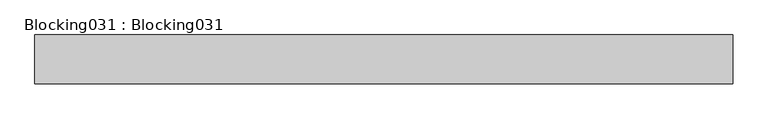
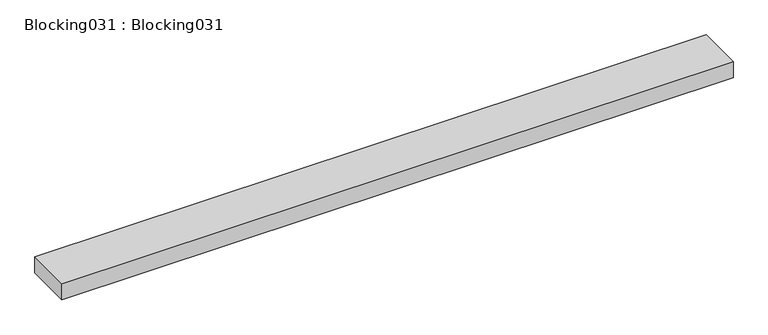
"""IFC4 building model written with IfcOpenShell, lengths in millimetres: proxy geometry, Blocking031 : Blocking031."""

from ifc_helpers import new_model, si_unit, frame, origin, place, context, project, spatial, polyline, outline, extrude, source, transform, mapped, element, save


def blocking031_blocking031_27079cb5(model_context):
    return source(origin(), model_context, "Body", "SweptSolid", [
        extrude(outline(polyline([(14383.0178845, -4497.8425368), (14383.0178845, -4637.5425368), (12383.0178845, -4637.5425368), (12383.0178845, -4497.8425368), (14383.0178845, -4497.8425368)])), frame((0.0, 0.0, 39706.296), z_axis=(0.0, 0.0, 1.0), x_axis=(1.0, 0.0, 0.0)), (0.0, 0.0, 1.0), 50.8),
    ])


if __name__ == "__main__":
    model = new_model("IFC4")
    model_context = context("Model", 3, world=origin())
    ifc_project = project(units=[si_unit("LENGTHUNIT", "METRE", prefix="MILLI")], contexts=[model_context])
    site = spatial("IfcSite", under=ifc_project)
    building = spatial("IfcBuilding", under=site)
    placement = place(None, origin())
    blocking031_blocking031_shape = blocking031_blocking031_27079cb5(model_context)
    element("IfcBuildingElementProxy", 1, Name="Blocking031 : Blocking031", ObjectType="Blocking031 : Blocking031", at=placement, inside=building, context=model_context, shape_type="MappedRepresentation", body=[
        mapped(blocking031_blocking031_shape, transform((0.0, 0.0, 0.0), x_axis=(1.0, 0.0, 0.0), y_axis=(0.0, 1.0, 0.0), z_axis=(0.0, 0.0, 1.0))),
    ])
    save(model, "model.ifc")

# Revit data of these elements
# Type "Blocking031 : Blocking031"
#   NameOverride = "Blocking031"
# Element 1 (IfcBuildingElementProxy, "Blocking031 : Blocking031")
#   Materials on its faces: "WOOD BLOCKING AS REQUIRED"
# Materials
#   "WOOD BLOCKING AS REQUIRED": class "Unassigned", colour RGB 166 124 85, transparency 0, Cost = 0
